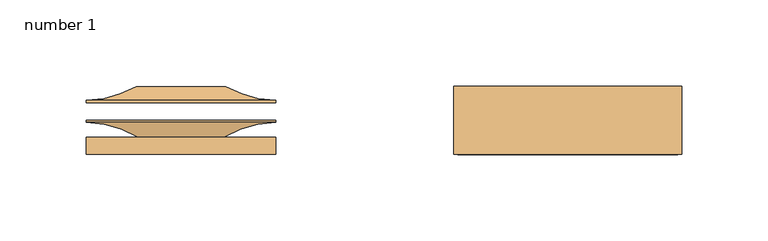
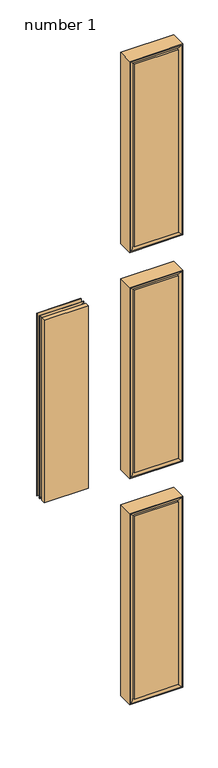
# IFC4 building model written with IfcOpenShell, lengths in millimetres: door geometry, Door-Interior-Karona-K5660-6_Panel : number 1.
# Revit data of these elements (continued)
# Type "Door-Interior-Karona-K5660-6_Panel : number 1" (continued)
#   Daylight Opening Height = 0' - 0"
#   Bottom Rail Height = 0' - 8 1/2"
#   3D Open Angle = 0.00°
#   Thickness = 0' - 1 3/4"
#   Stop Thickness = 0' - 0 1/2"
#   Stop Depth = 0' - 1 3/8"
#   Rough Width = 2' - 1 29/32"
#   Rough Height = 6' - 8 61/64"
#   Rabbet Width = 0' - 1 3/4"
#   Jamb Offset = 0' - 0 61/64"
#   Hinge Offset = 0' - 0 3/4"
#   Jamb Thickness = 0' - 0 29/32"
#   Ext. Frame Thickness = 0' - 0 5/8"
#   Int. Frame Thickness = 0' - 0 5/8"
#   Height = 6' - 8"
#   Width = 2' - 0"
#   3D Angle = 0.00°
#   Trim Visible = yes
#   Square Sticking Profile = no
#   Raised Panel Door = yes
#   Ovolo Sticking Profile = yes
#   Ogee Sticking Profile = no
#   Mission Sticking Profile = no
#   Hinge Visible = yes
#   Glass Panel Door = no
#   Flat Panel Door = no
#   Edition number = 1
#   Define Thermal Properties by = 1
#   Trim Material = Wood - Karona - Red Oak
#   Top Rail Material = Wood - Karona - Red Oak
#   Stile Material = Wood - Karona - Red Oak
#   Sticking Material = Wood - Karona - Red Oak
#   Jamb Material = Wood - Karona - Red Oak
#   Interior Panel = Wood - Karona - Red Oak
#   Door Panel Material = Wood - Karona - Red Oak
#   Bottom Rail Material = Wood - Karona - Red Oak
#   Visual Light Transmittance = 0
#   Solar Heat Gain Coefficient = 0
#   Construction Type = (empty or 0)
#   Function = (empty or 0)
#   Wall Closure = (empty or 0)
# Element 1 (IfcDoor, "Door-Interior-Karona-K5660-6_Panel : number 1")
#   Materials on its faces: "Wood - Karona - Red Oak"
# Materials
#   "Wood - Karona - Red Oak": class "Wood", colour RGB 153 121 89, transparency 0, Description = "Quercus Rubra", Cost = 0
